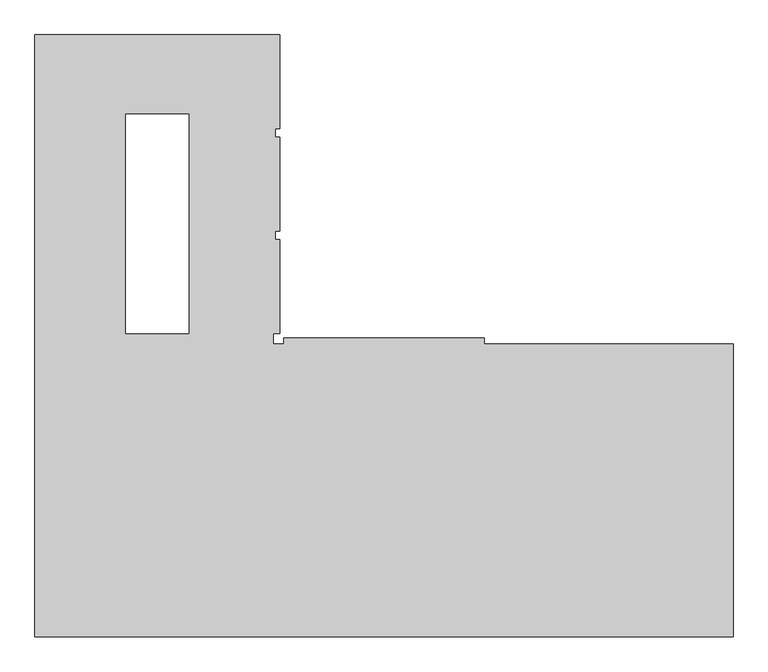
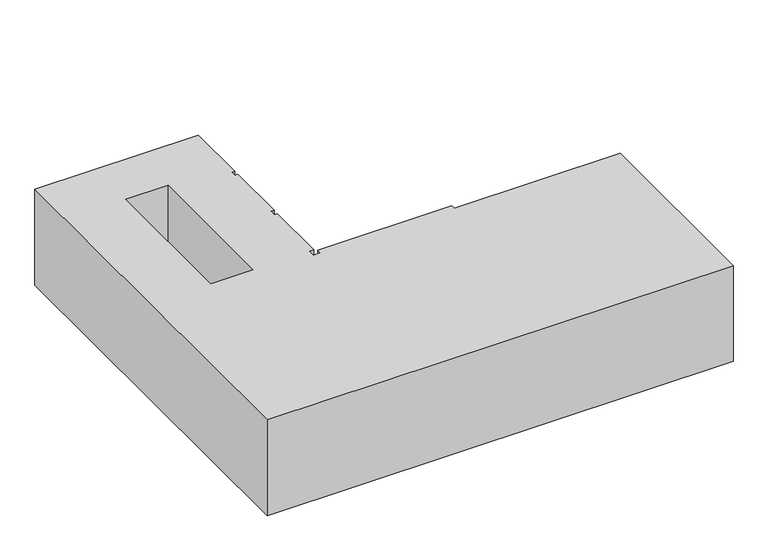
"""IFC4 building model written with IfcOpenShell, lengths in millimetres: proxy geometry, 0_3d."""

from ifc_helpers import new_model, si_unit, origin, origin_with_axes, place, context, project, spatial, polyline, outline, extrude, source, transform, mapped, element, save


def generic_models_af74dbcd(model_context):
    return source(origin(), model_context, "Body", "SweptSolid", [
        extrude(outline(polyline([(4520.0, 5552.8619019), (4720.0, 5552.8619019), (4720.0, 5674.8619019), (8520.0, 5674.8619019), (8520.0, 5552.8619019), (13240.0, 5552.8619019), (13240.0, 0.0), (0.0, 0.0), (0.0, 11422.8619019), (4642.0, 11422.8619019), (4642.0, 9639.4619019), (4560.0, 9639.4619019), (4560.0, 9479.4619019), (4642.0, 9479.4619019), (4642.0, 7696.1619019), (4560.0, 7696.1619019), (4560.0, 7536.1619019), (4642.0, 7536.1619019), (4642.0, 5752.8619019), (4520.0, 5752.8619019), (4520.0, 5552.8619019)]), holes=[polyline([(1718.7090817, 5752.8619019), (2919.4613155, 5752.8619019), (2919.4613155, 9922.8619019), (1718.7090817, 9922.8619019), (1718.7090817, 5752.8619019)])]), origin_with_axes(), (0.0, 0.0, 1.0), 2880.0),
    ])


if __name__ == "__main__":
    model = new_model("IFC4")
    model_context = context("Model", 3, world=origin())
    ifc_project = project(units=[si_unit("LENGTHUNIT", "METRE", prefix="MILLI")], contexts=[model_context])
    site = spatial("IfcSite", under=ifc_project)
    building = spatial("IfcBuilding", under=site)
    placement = place(None, origin())
    generic_models_shape = generic_models_af74dbcd(model_context)
    element("IfcBuildingElementProxy", 1, Name="0_3d", ObjectType="0_3d", at=placement, inside=building, context=model_context, shape_type="MappedRepresentation", body=[
        mapped(generic_models_shape, transform((0.0, 0.0, 0.0), x_axis=(1.0, 0.0, 0.0), y_axis=(0.0, 1.0, 0.0), z_axis=(0.0, 0.0, 1.0))),
    ])
    save(model, "model.ifc")

# Revit data of these elements
# Element 1 (IfcBuildingElementProxy, "0_3d")
#   Materials on its faces: "*1"
# Materials
#   "*1": class "Unassigned", colour RGB 175 175 175, transparency 0
